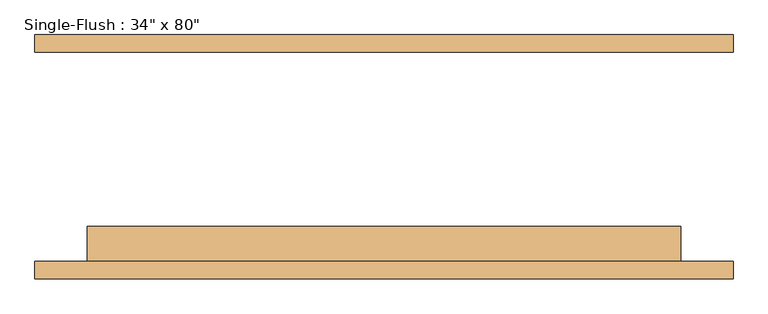
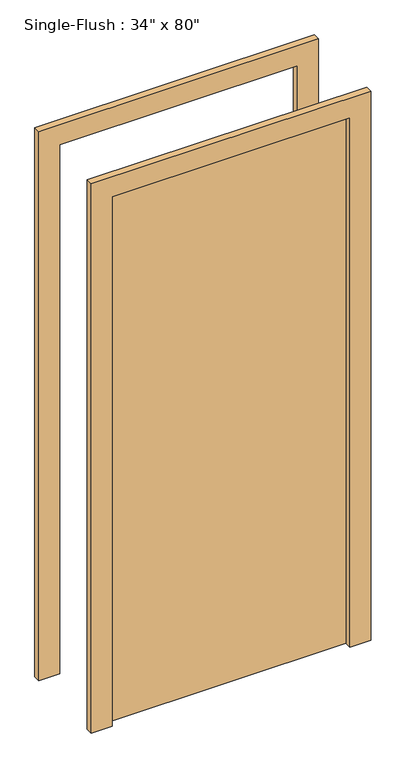
"""IFC4 building model written with IfcOpenShell, lengths in millimetres: door geometry."""

from ifc_helpers import new_model, si_unit, frame, origin, origin_with_axes, place, context, project, spatial, polyline, outline, extrude, source, transform, mapped, element, save


def door_573a7c88(model_context):
    return source(origin(), model_context, "Body", "SweptSolid", [
        extrude(outline(polyline([(2108.2, -508.0), (0.0, -508.0), (0.0, -431.8), (2032.0, -431.8), (2032.0, 431.8), (0.0, 431.8), (0.0, 508.0), (2108.2, 508.0), (2108.2, -508.0)])), frame((0.0, -177.8, 0.0), z_axis=(0.0, 1.0, 0.0), x_axis=(0.0, 0.0, 1.0)), (0.0, 0.0, 1.0), 25.4),
        extrude(outline(polyline([(2108.2, 508.0), (2108.2, -508.0), (0.0, -508.0), (0.0, -431.8), (2032.0, -431.8), (2032.0, 431.8), (0.0, 431.8), (0.0, 508.0), (2108.2, 508.0)])), frame((0.0, 152.4, 0.0), z_axis=(0.0, 1.0, 0.0), x_axis=(0.0, 0.0, 1.0)), (0.0, 0.0, 1.0), 25.4),
        extrude(outline(polyline([(431.8, -101.6), (431.8, -152.4), (-431.8, -152.4), (-431.8, -101.6), (431.8, -101.6)])), origin_with_axes(), (0.0, 0.0, 1.0), 2032.0),
    ])


if __name__ == "__main__":
    model = new_model("IFC4")
    model_context = context("Model", 3, world=origin())
    ifc_project = project(units=[si_unit("LENGTHUNIT", "METRE", prefix="MILLI")], contexts=[model_context])
    site = spatial("IfcSite", under=ifc_project)
    building = spatial("IfcBuilding", under=site)
    placement = place(None, origin())
    door_shape = door_573a7c88(model_context)
    element("IfcDoor", 1, ObjectType="Single-Flush : 34\" x 80\"", at=placement, inside=building, context=model_context, shape_type="MappedRepresentation", body=[
        mapped(door_shape, transform((0.0, 0.0, 0.0), x_axis=(1.0, 0.0, 0.0), y_axis=(0.0, 1.0, 0.0), z_axis=(0.0, 0.0, 1.0))),
    ])
    save(model, "model.ifc")

# Revit data of these elements
# Type "Single-Flush : 34\" x 80\""
#   Type Mark = "7"
#   Construction Type Id = "MDOOR"
#   Assembly Code = "C1020"
#   Analytic Construction = "Metal"
#   Thickness = 0' - 2"
#   Heat Transfer Coefficient (U) = 0.651978 BTU/(h·ft²·°F)
#   Height = 6' - 8"
#   Trim Projection Ext = 0' - 1"
#   Trim Projection Int = 0' - 1"
#   Trim Width = 0' - 3"
#   Width = 2' - 10"
#   Define Thermal Properties by = 1
#   Define Thermal Properties by = 1
#   Door Material = Door - Panel
#   Frame Material = Door - Frame
#   Visual Light Transmittance = 0
#   Solar Heat Gain Coefficient = 0
#   Function = (empty or 0)
#   Wall Closure = (empty or 0)
# Element 1 (IfcDoor, "Single-Flush : 34\" x 80\"")
#   Materials on its faces: "Door - Frame", "Door - Panel"
# Materials
#   "Door - Panel": class "Wood", colour RGB 210 159 95, transparency 0, Cost = 0
#   "Door - Frame": class "Miscellaneous", colour RGB 118 70 51, transparency 0, Cost = 0
